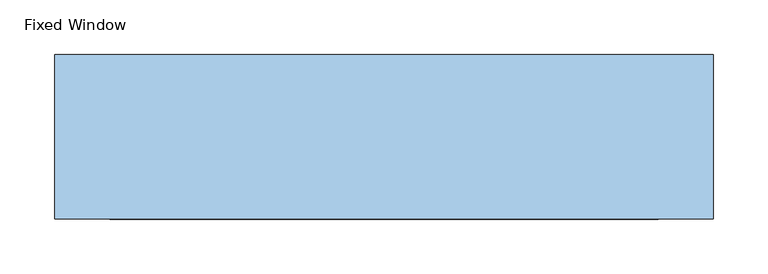
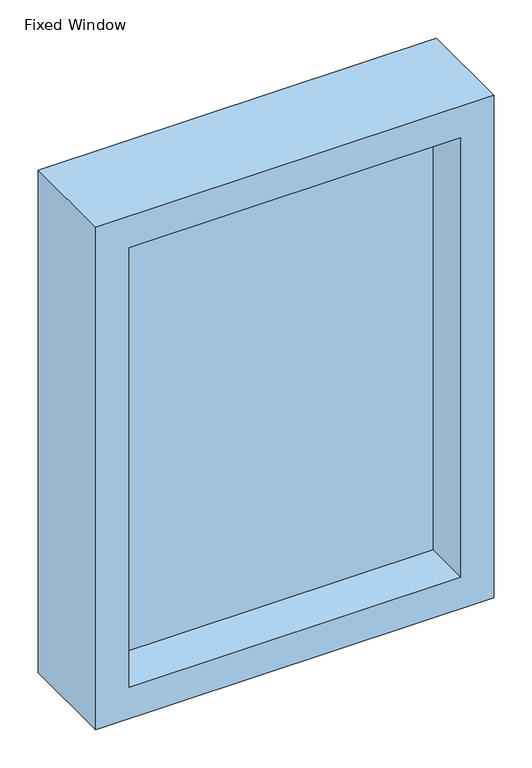
"""IFC4 building model written with IfcOpenShell, lengths in millimetres: window geometry, Fixed Window : H_WD_AMW_AL Window_DG_W600xH600_Fixed_1H1V."""

import ifcopenshell
import ifcopenshell.guid

model = None  # the IFC model being written
_history = None  # IfcOwnerHistory: only IFC2X3 demands one
_inside = {}  # id of a spatial element -> (the spatial element, [elements in it])
_under = {}  # id of a project, library or spatial element -> (it, [spatial elements below it])
_declared = {}  # id of a project -> (the project, [libraries it declares])
_typed = {}  # id of a type object -> (the type object, [elements of that type])
_made_of = {}  # id of a material, layer set ... -> (it, [elements and type objects made of it])


def new_model(schema):
    """Start an empty IFC model of exactly this schema.

    Asked for "IFC4X3", IfcOpenShell would pick the latest addendum, in which some entities
    have other attributes; the version numbers below select the first issue.
    IFC2X3 requires an IfcOwnerHistory on every rooted entity: one is made here for all.
    """
    global model, _history
    if schema == "IFC4X3":
        model = ifcopenshell.file(schema_version=(4, 3, 0, 0))
    else:
        model = ifcopenshell.file(schema=schema)
    _inside.clear()
    _under.clear()
    _declared.clear()
    _typed.clear()
    _made_of.clear()
    _history = None
    if model.schema == "IFC2X3":
        org = make("IfcOrganization", Name="unknown")
        user = make(
            "IfcPersonAndOrganization",
            ThePerson=make("IfcPerson", FamilyName="unknown"),
            TheOrganization=org,
        )
        app = make(
            "IfcApplication",
            ApplicationDeveloper=org,
            Version="unknown",
            ApplicationFullName="unknown",
            ApplicationIdentifier="unknown",
        )
        _history = make(
            "IfcOwnerHistory",
            OwningUser=user,
            OwningApplication=app,
            ChangeAction="ADDED",
            CreationDate=0,
        )
    return model


def make(cls, **values):
    """One entity of the class cls with the attributes given. An attribute that is None is left unset."""
    return model.create_entity(
        cls, **{name: value for name, value in values.items() if value is not None}
    )


def rooted(cls, **values):
    """An entity with a GlobalId (a new one), such as an element, a storey or a relation."""
    return make(cls, GlobalId=ifcopenshell.guid.new(), OwnerHistory=_history, **values)


def si_unit(unit_type, name, prefix=None):
    """IfcSIUnit, for example si_unit("LENGTHUNIT", "METRE", prefix="MILLI")."""
    return make("IfcSIUnit", UnitType=unit_type, Prefix=prefix, Name=name)


def assignment(units):
    """IfcUnitAssignment: the units of a project."""
    return None if units is None else make("IfcUnitAssignment", Units=units)


def point(xyz):
    """IfcCartesianPoint."""
    return None if xyz is None else make("IfcCartesianPoint", Coordinates=xyz)


def direction(xyz):
    """IfcDirection."""
    return None if xyz is None else make("IfcDirection", DirectionRatios=xyz)


def frame(location, z_axis=None, x_axis=None):
    """IfcAxis2Placement3D, a coordinate frame: its origin and axes. An axis left out is left unset."""
    return make(
        "IfcAxis2Placement3D",
        Location=point(location),
        Axis=direction(z_axis),
        RefDirection=direction(x_axis),
    )


def origin():
    """The frame at (0, 0, 0) with its axes left unset."""
    return frame((0.0, 0.0, 0.0))


def place(relative_to, where):
    """IfcLocalPlacement: puts the frame where relative to a parent placement (None: the world)."""
    return make(
        "IfcLocalPlacement", PlacementRelTo=relative_to, RelativePlacement=where
    )


def context(
    kind, dimensions, precision=None, world=None, true_north=None, identifier=None
):
    """IfcGeometricRepresentationContext, for example the 3D "Model" context."""
    return make(
        "IfcGeometricRepresentationContext",
        ContextIdentifier=identifier,
        ContextType=kind,
        CoordinateSpaceDimension=dimensions,
        Precision=precision,
        WorldCoordinateSystem=world,
        TrueNorth=true_north,
    )


def project(units=None, contexts=None):
    """IfcProject with its units and contexts."""
    return rooted(
        "IfcProject",
        Name="project",
        RepresentationContexts=contexts,
        UnitsInContext=assignment(units),
    )


def spatial(cls, under=None, at=None, **own):
    """A site, building, storey or space (cls), placed at a placement, below another one or the project."""
    s = rooted(cls, ObjectPlacement=at, **own)
    if under is not None:
        _under.setdefault(under.id(), (under, []))[1].append(s)
    return s


def polyline(points):
    """IfcPolyline through the points."""
    return make("IfcPolyline", Points=[point(p) for p in points])


def outline(outer, holes=None, kind="AREA"):
    """IfcArbitraryClosedProfileDef: a profile drawn as a closed curve; with holes, ...WithVoids."""
    if holes is None:
        return make("IfcArbitraryClosedProfileDef", ProfileType=kind, OuterCurve=outer)
    return make(
        "IfcArbitraryProfileDefWithVoids",
        ProfileType=kind,
        OuterCurve=outer,
        InnerCurves=holes,
    )


def extrude(swept, where, along, depth):
    """IfcExtrudedAreaSolid: the profile swept, set in the frame where, extruded along a direction by depth."""
    return make(
        "IfcExtrudedAreaSolid",
        SweptArea=swept,
        Position=where,
        ExtrudedDirection=direction(along),
        Depth=depth,
    )


def shape(context_of_items, identifier, shape_type, items):
    """IfcShapeRepresentation: the items that make up one representation, for example the "Body"."""
    return make(
        "IfcShapeRepresentation",
        ContextOfItems=context_of_items,
        RepresentationIdentifier=identifier,
        RepresentationType=shape_type,
        Items=items,
    )


def source(mapping_origin, context_of_items, identifier, shape_type, items):
    """IfcRepresentationMap: a shape defined once, which mapped items show again and again."""
    return make(
        "IfcRepresentationMap",
        MappingOrigin=mapping_origin,
        MappedRepresentation=shape(context_of_items, identifier, shape_type, items),
    )


def transform(
    local_origin,
    x_axis=None,
    y_axis=None,
    z_axis=None,
    scale=None,
    scale2=None,
    scale3=None,
    uniform=True,
):
    """IfcCartesianTransformationOperator3D, or its non-uniform kind. x_axis, y_axis, z_axis: its Axis1, 2, 3."""
    if uniform:
        return make(
            "IfcCartesianTransformationOperator3D",
            Axis1=direction(x_axis),
            Axis2=direction(y_axis),
            LocalOrigin=point(local_origin),
            Scale=scale,
            Axis3=direction(z_axis),
        )
    return make(
        "IfcCartesianTransformationOperator3DnonUniform",
        Axis1=direction(x_axis),
        Axis2=direction(y_axis),
        LocalOrigin=point(local_origin),
        Scale=scale,
        Axis3=direction(z_axis),
        Scale2=scale2,
        Scale3=scale3,
    )


def mapped(mapping_source, mapping_target):
    """IfcMappedItem: shows the shape of a source again, moved by a transform."""
    return make(
        "IfcMappedItem", MappingSource=mapping_source, MappingTarget=mapping_target
    )


def made_of(thing, what):
    """Note that an element or type object is made of a material, layer set ...; save() writes the relation."""
    if what is not None:
        _made_of.setdefault(what.id(), (what, []))[1].append(thing)
    return thing


def element(
    cls,
    number,
    at=None,
    inside=None,
    cuts=None,
    type_object=None,
    material=None,
    context=None,
    identifier="Body",
    shape_type=None,
    held_by="IfcProductDefinitionShape",
    body=None,
    shapes=None,
    **own,
):
    """One element of the class cls, such as IfcWall. Its Tag is "e" and its number.

    at: its placement. inside: the storey or other place that contains it. cuts: it is an
    opening in that element (IfcRelVoidsElement). A single representation is given by context,
    identifier, shape_type and body (its items); several are given by shapes. held_by: the class
    of the entity that holds the representations. save() writes the other relations.
    """
    e = rooted(cls, Tag="e%d" % number, ObjectPlacement=at, **own)
    if body is not None:
        shapes = [shape(context, identifier, shape_type, body)]
    if shapes is not None:
        e.Representation = make(held_by, Representations=shapes)
    if inside is not None:
        _inside.setdefault(inside.id(), (inside, []))[1].append(e)
    if cuts is not None:
        rooted(
            "IfcRelVoidsElement", RelatingBuildingElement=cuts, RelatedOpeningElement=e
        )
    if type_object is not None:
        _typed.setdefault(type_object.id(), (type_object, []))[1].append(e)
    return made_of(e, material)


def aggregate(whole, parts):
    """IfcRelAggregates: a whole, such as a stair, and the parts it consists of."""
    return rooted("IfcRelAggregates", RelatingObject=whole, RelatedObjects=parts)


def save(model, path):
    """Write the relations noted so far, then the file.

    IfcRelAggregates (storeys below a building ...), IfcRelContainedInSpatialStructure (elements
    in a storey), IfcRelDefinesByType, IfcRelAssociatesMaterial and IfcRelDeclares: one each for
    every whole, place, type object, material and project.
    """
    for whole, parts in _under.values():
        aggregate(whole, parts)
    for where, things in _inside.values():
        rooted(
            "IfcRelContainedInSpatialStructure",
            RelatedElements=things,
            RelatingStructure=where,
        )
    for kind, things in _typed.values():
        rooted("IfcRelDefinesByType", RelatedObjects=things, RelatingType=kind)
    for what, things in _made_of.values():
        rooted("IfcRelAssociatesMaterial", RelatedObjects=things, RelatingMaterial=what)
    for by, libraries in _declared.values():
        rooted("IfcRelDeclares", RelatingContext=by, RelatedDefinitions=libraries)
    model.write(path)


def fixed_window_37dd25d6(model_context):
    return source(origin(), model_context, "Body", "SweptSolid", [
        extrude(outline(polyline([(-250.0, 3.0), (250.0, 3.0), (250.0, -3.0), (-250.0, -3.0), (-250.0, 3.0)])), frame((0.0, 0.0, 850.0), z_axis=(0.0, 0.0, 1.0), x_axis=(1.0, 0.0, 0.0)), (0.0, 0.0, 1.0), 700.0),
        extrude(outline(polyline([(1600.0, -300.0), (800.0, -300.0), (800.0, 300.0), (1600.0, 300.0), (1600.0, -300.0)]), holes=[polyline([(1550.0, -250.0), (1550.0, 250.0), (850.0, 250.0), (850.0, -250.0), (1550.0, -250.0)])]), frame((0.0, -75.0, 0.0), z_axis=(0.0, 1.0, 0.0), x_axis=(0.0, 0.0, 1.0)), (0.0, 0.0, 1.0), 150.0),
    ])


if __name__ == "__main__":
    model = new_model("IFC4")
    model_context = context("Model", 3, world=origin())
    ifc_project = project(units=[si_unit("LENGTHUNIT", "METRE", prefix="MILLI")], contexts=[model_context])
    site = spatial("IfcSite", under=ifc_project)
    building = spatial("IfcBuilding", under=site)
    placement = place(None, origin())
    fixed_window_shape = fixed_window_37dd25d6(model_context)
    element("IfcWindow", 1, ObjectType="Fixed Window : H_WD_AMW_AL Window_DG_W600xH600_Fixed_1H1V", at=placement, inside=building, context=model_context, shape_type="MappedRepresentation", body=[
        mapped(fixed_window_shape, transform((0.0, 0.0, 0.0), x_axis=(1.0, 0.0, 0.0), y_axis=(0.0, 1.0, 0.0), z_axis=(0.0, 0.0, 1.0))),
    ])
    save(model, "model.ifc")

# Revit data of these elements
# Type "Fixed Window : H_WD_AMW_AL Window_DG_W600xH600_Fixed_1H1V"
#   Type Mark = "AW"
#   Analytic Construction = "<None>"
#   창 두께 = 0.1500 m
#   Height = 0.8000 m
#   절반 창 두께 = 0.0750 m
#   기본 씰 높이 = 0.8000 m
#   Width = 0.6000 m
#   Define Thermal Properties by = 1
#   창 패널 = AW2 창 패널
#   창 프레임 = A04AQ127-00002_Aluminum Window_None FP
#   Wall Closure = (empty or 0)
# Element 1 (IfcWindow, "Fixed Window : H_WD_AMW_AL Window_DG_W600xH600_Fixed_1H1V")
#   Materials on its faces: "A04AQ127-00002_Aluminum Window_None FP", "AW2 창 패널"
# Materials
#   "AW2 창 패널": class "유리", colour RGB 0 0 255, transparency 0.75
#   "A04AQ127-00002_Aluminum Window_None FP": class "금속", colour RGB 247 247 247, transparency 0, Cost = 0
